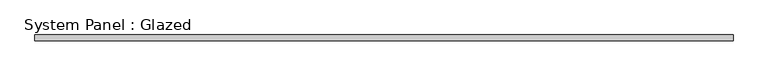
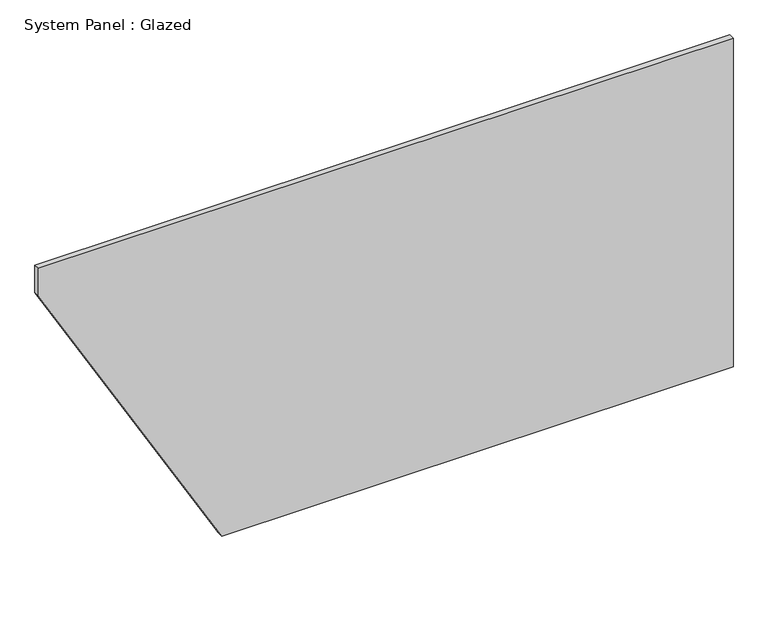
"""IFC4 building model written with IfcOpenShell, lengths in millimetres: plate geometry, System Panel : Glazed."""

from ifc_helpers import new_model, si_unit, frame, origin, place, context, project, spatial, polyline, outline, extrude, source, transform, mapped, element, save


def system_panel_glazed_b0066566(model_context):
    return source(origin(), model_context, "Body", "SweptSolid", [
        extrude(outline(polyline([(0.0, -708.1404747), (0.0, 1500.0), (1500.0, 1500.0), (1500.0, -1500.0), (1372.5184302, -1500.0), (0.0, -708.1404747)])), frame((0.0, 24.5, 0.0), z_axis=(0.0, 1.0, 0.0), x_axis=(0.0, 0.0, 1.0)), (0.0, 0.0, 1.0), 25.0),
    ])


if __name__ == "__main__":
    model = new_model("IFC4")
    model_context = context("Model", 3, world=origin())
    ifc_project = project(units=[si_unit("LENGTHUNIT", "METRE", prefix="MILLI")], contexts=[model_context])
    site = spatial("IfcSite", under=ifc_project)
    building = spatial("IfcBuilding", under=site)
    placement = place(None, origin())
    system_panel_glazed_shape = system_panel_glazed_b0066566(model_context)
    element("IfcPlate", 1, ObjectType="System Panel : Glazed", at=placement, inside=building, context=model_context, shape_type="MappedRepresentation", body=[
        mapped(system_panel_glazed_shape, transform((0.0, 0.0, 0.0), x_axis=(1.0, 0.0, 0.0), y_axis=(0.0, 1.0, 0.0), z_axis=(0.0, 0.0, 1.0))),
    ])
    save(model, "model.ifc")

# Revit data of these elements
# Type "System Panel : Glazed"
#   Construction Type Id = "GSP4R"
#   Analytic Construction = "1/8 in Pilkington single glazing"
#   Visual Light Transmittance = 0.9
#   Solar Heat Gain Coefficient = 0.86
#   Heat Transfer Coefficient (U) = 6.7069 W/(m²·K)
#   Define Thermal Properties by = 1
# Element 1 (IfcPlate, "System Panel : Glazed")
#   Materials on its faces: "Glass"
# Materials
#   "Glass": class "Glass", colour RGB 0 128 192, transparency 0.9, Description = "Soda Lime Glass", Cost = 0
